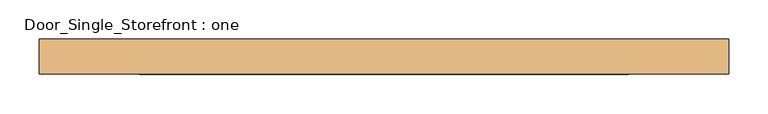
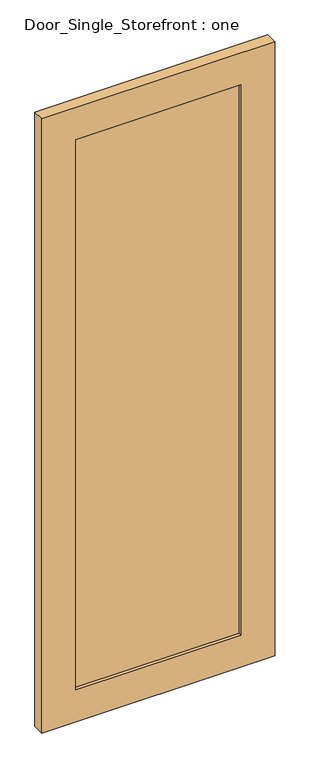
"""IFC4 building model written with IfcOpenShell, lengths in millimetres: door geometry, Door_Single_Storefront : one."""

from ifc_helpers import new_model, si_unit, frame, origin, place, context, project, spatial, polyline, outline, extrude, source, transform, mapped, element, save


def door_single_storefront_one_1daa2e39(model_context):
    return source(origin(), model_context, "Body", "SweptSolid", [
        extrude(outline(polyline([(310.35625, -6.35), (-310.35625, -6.35), (-310.35625, 12.7), (310.35625, 12.7), (310.35625, -6.35)])), frame((0.0, 0.0, 127.0), z_axis=(0.0, 0.0, 1.0), x_axis=(1.0, 0.0, 0.0)), (0.0, 0.0, 1.0), 2184.4),
        extrude(outline(polyline([(2438.4, -437.35625), (0.0, -437.35625), (0.0, 437.35625), (2438.4, 437.35625), (2438.4, -437.35625)]), holes=[polyline([(127.0, 310.35625), (127.0, -310.35625), (2311.4, -310.35625), (2311.4, 310.35625), (127.0, 310.35625)])]), frame((0.0, -19.05, 0.0), z_axis=(0.0, 1.0, 0.0), x_axis=(0.0, 0.0, 1.0)), (0.0, 0.0, 1.0), 44.45),
    ])


if __name__ == "__main__":
    model = new_model("IFC4")
    model_context = context("Model", 3, world=origin())
    ifc_project = project(units=[si_unit("LENGTHUNIT", "METRE", prefix="MILLI")], contexts=[model_context])
    site = spatial("IfcSite", under=ifc_project)
    building = spatial("IfcBuilding", under=site)
    placement = place(None, origin())
    door_single_storefront_one_shape = door_single_storefront_one_1daa2e39(model_context)
    element("IfcDoor", 1, ObjectType="Door_Single_Storefront : one", at=placement, inside=building, context=model_context, shape_type="MappedRepresentation", body=[
        mapped(door_single_storefront_one_shape, transform((0.0, 0.0, 0.0), x_axis=(1.0, 0.0, 0.0), y_axis=(0.0, 1.0, 0.0), z_axis=(0.0, 0.0, 1.0))),
    ])
    save(model, "model.ifc")

# Revit data of these elements
# Type "Door_Single_Storefront : one"
#   Type Mark = "27"
#   Analytic Construction = "<None>"
#   Stile_Width = 0' - 5"
#   Door_Thickness = 0' - 1 3/4"
#   Door_Offset = 0' - 1"
#   Glass_Material = SAFETY GLAZING
#   Frame_Material = INTERIOR GRADE ALUMINUM STOREFRONT W/ SAFETY GLAZING
#   Function = (empty or 0)
# Element 1 (IfcDoor, "Door_Single_Storefront : one")
#   Materials on its faces: "INTERIOR GRADE ALUMINUM STOREFRONT W/ SAFETY GLAZING", "SAFETY GLAZING"
# Materials
#   "SAFETY GLAZING": class "Glass", colour RGB 142 168 196, transparency 0.75, Description = "Soda Lime Glass", Cost = 0
#   "INTERIOR GRADE ALUMINUM STOREFRONT W/ SAFETY GLAZING": class "Metal", colour RGB 226 226 226, transparency 0, Description = "Aluminum 6061", Cost = 0
